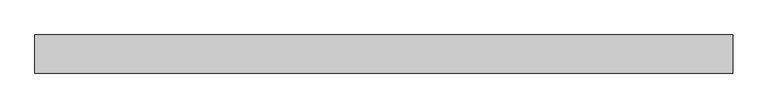
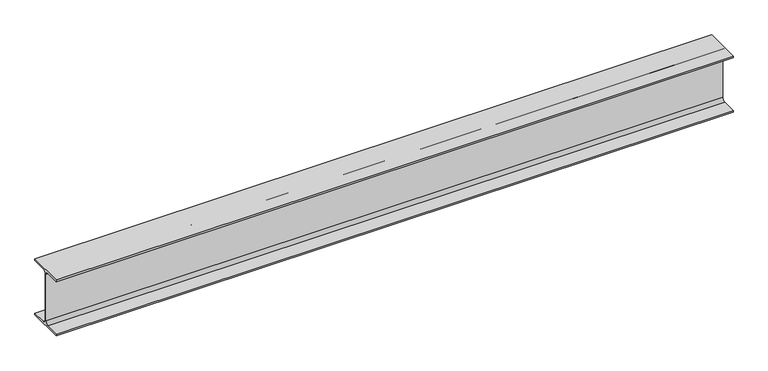
"""IFC4 building model written with IfcOpenShell, lengths in millimetres: beam geometry, 0912_Steel Framing_H-KSD3502 : H_SB_ASB_H-482x300x11x15."""

from ifc_helpers import new_model, si_unit, point, frame, frame_2d, origin, place, context, project, spatial, polyline, circle_curve, trimmed, segment, composite_curve, outline, extrude, source, transform, mapped, element, save


def beam_68c26b3c(model_context):
    return source(origin(), model_context, "Body", "SweptSolid", [
        extrude(outline(composite_curve([segment(polyline([(150.0, -226.0), (150.0, -241.0), (-150.0, -241.0), (-150.0, -226.0), (-31.5, -226.0)]), True, "CONTINUOUS"), segment(trimmed(circle_curve(frame_2d((-31.5, -200.0)), 26.0), [point((-31.5, -226.0))], [point((-5.5, -200.0))], True, "CARTESIAN"), True, "CONTINUOUS"), segment(polyline([(-5.5, -200.0), (-5.5, 200.0)]), True, "CONTINUOUS"), segment(trimmed(circle_curve(frame_2d((-31.5, 200.0)), 26.0), [point((-5.5, 200.0))], [point((-31.5, 226.0))], True, "CARTESIAN"), True, "CONTINUOUS"), segment(polyline([(-31.5, 226.0), (-150.0, 226.0), (-150.0, 241.0), (150.0, 241.0), (150.0, 226.0), (31.5, 226.0)]), True, "CONTINUOUS"), segment(trimmed(circle_curve(frame_2d((31.5, 200.0)), 26.0), [point((31.5, 226.0))], [point((5.5, 200.0))], True, "CARTESIAN"), True, "CONTINUOUS"), segment(polyline([(5.5, 200.0), (5.5, -200.0)]), True, "CONTINUOUS"), segment(trimmed(circle_curve(frame_2d((31.5, -200.0)), 26.0), [point((5.5, -200.0))], [point((31.5, -226.0))], True, "CARTESIAN"), True, "CONTINUOUS"), segment(polyline([(31.5, -226.0), (150.0, -226.0)]), True, "CONTINUOUS")], self_intersect=False)), frame((-2662.3, 0.0, 0.0), z_axis=(1.0, 0.0, 0.0), x_axis=(0.0, 1.0, 0.0)), (0.0, 0.0, 1.0), 5487.3),
    ])


if __name__ == "__main__":
    model = new_model("IFC4")
    model_context = context("Model", 3, world=origin())
    ifc_project = project(units=[si_unit("LENGTHUNIT", "METRE", prefix="MILLI")], contexts=[model_context])
    site = spatial("IfcSite", under=ifc_project)
    building = spatial("IfcBuilding", under=site)
    placement = place(None, origin())
    beam_shape = beam_68c26b3c(model_context)
    element("IfcBeam", 1, ObjectType="0912_Steel Framing_H-KSD3502 : H_SB_ASB_H-482x300x11x15", at=placement, inside=building, context=model_context, shape_type="MappedRepresentation", body=[
        mapped(beam_shape, transform((0.0, 0.0, 0.0), x_axis=(1.0, 0.0, 0.0), y_axis=(0.0, 1.0, 0.0), z_axis=(0.0, 0.0, 1.0))),
    ])
    save(model, "model.ifc")

# Revit data of these elements
# Type "0912_Steel Framing_H-KSD3502 : H_SB_ASB_H-482x300x11x15"
#   H_WM Code_1 = "S01AA001-00001 | Main Steel Structure Fabrication Work | Shelter/Building | Heavy Steel - Standard (Weight≥90KG/M) | Material: (   )"
#   H_WM Code_2 = "S03AA027-00001 | Main Steel Structure Erection Work | Shelter/Building | Heavy Steel (Weight≥90KG/M) | Material: (   )"
#   H_WM Code_3 = "S01AA010-00001 | Main Steel Structure Fabrication Work | Shelter/Building | Steel Painting/Coating | for Non-Fireproofed Steel Surface, Surface Preparation, Primer, Second & Final Coat | Material: (   )"
#   H_Q'ty Cal Type Tag = "SB-Q2"
#   Width = 30.0 cm
#   Web Thickness = 1.1 cm
#   Web Fillet = 2.6 cm
#   Warping Constant = 3680000.0 cm⁶
#   W = 0
#   Torsional Moment of Inertia = 88.2192 cm⁴
#   Section Area = 145.5 cm²
#   Plastic Modulus weak axis = 695.0 cm³
#   Plastic Modulus strong axis = 2790.0 cm³
#   Perimeter = 2.10 m²/m
#   Nominal Weight = 114.00 kgf/m
#   Moment of Inertia weak axis = 6760.00 cm⁴
#   Moment of Inertia strong axis = 60400.00 cm⁴
#   Height = 48.2 cm
#   Flange Thickness = 1.5 cm
#   Elastic Modulus weak axis = 451.0 cm³
#   Elastic Modulus strong axis = 2500.0 cm³
#   Centroid Vertical = 24.1 cm
#   Centroid Horizontal = 15.0 cm
#   Ix = 604000000
#   Length [instance default] = 1.5240 m
#   Zx = 2790000
#   b = 0.3000 m
#   h = 0.4820 m
#   r = 0.0260 m
#   s = 0.0110 m
#   t = 0.0150 m
#   A = 0.01455 m²
#   Structural Material [instance default] = Steel, 45-345
#   Assembly Code = ""
# Element 1 (IfcBeam, "0912_Steel Framing_H-KSD3502 : H_SB_ASB_H-482x300x11x15")
#   Structural Material = none
# Materials
#   "Steel, 45-345": class "Metal", colour RGB 189 187 185, transparency 0, Description = "Steel 345 MPa", Cost = 0
